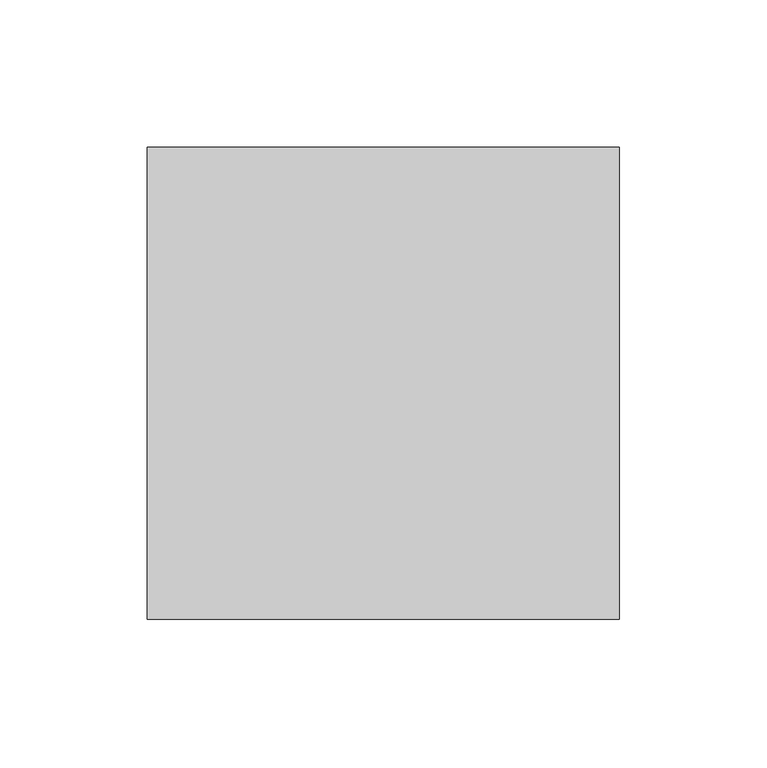
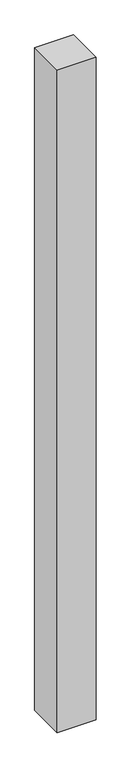
"""IFC4 building model written with IfcOpenShell, lengths in millimetres: proxy geometry, 0_3d."""

from ifc_helpers import new_model, si_unit, origin, origin_with_axes, place, context, project, spatial, polyline, outline, extrude, source, transform, mapped, element, save


def generic_models_cc99bfa8(model_context):
    return source(origin(), model_context, "Body", "SweptSolid", [
        extrude(outline(polyline([(159076.7593015, 40464.7962965), (159076.7593015, 40304.7962965), (158916.7593015, 40304.7962965), (158916.7593015, 40464.7962965), (159076.7593015, 40464.7962965)])), origin_with_axes(), (0.0, 0.0, 1.0), 2880.0),
    ])


if __name__ == "__main__":
    model = new_model("IFC4")
    model_context = context("Model", 3, world=origin())
    ifc_project = project(units=[si_unit("LENGTHUNIT", "METRE", prefix="MILLI")], contexts=[model_context])
    site = spatial("IfcSite", under=ifc_project)
    building = spatial("IfcBuilding", under=site)
    placement = place(None, origin())
    generic_models_shape = generic_models_cc99bfa8(model_context)
    element("IfcBuildingElementProxy", 1, Name="0_3d", ObjectType="0_3d", at=placement, inside=building, context=model_context, shape_type="MappedRepresentation", body=[
        mapped(generic_models_shape, transform((0.0, 0.0, 0.0), x_axis=(1.0, 0.0, 0.0), y_axis=(0.0, 1.0, 0.0), z_axis=(0.0, 0.0, 1.0))),
    ])
    save(model, "model.ifc")

# Revit data of these elements
# Element 1 (IfcBuildingElementProxy, "0_3d")
#   Materials on its faces: "material wardrobe b 1"
# Materials
#   "material wardrobe b 1": class "Unassigned", colour RGB 128 128 128, transparency 0
